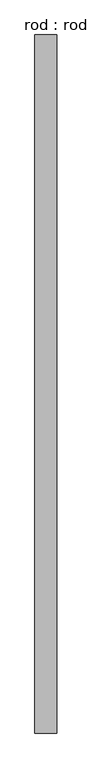
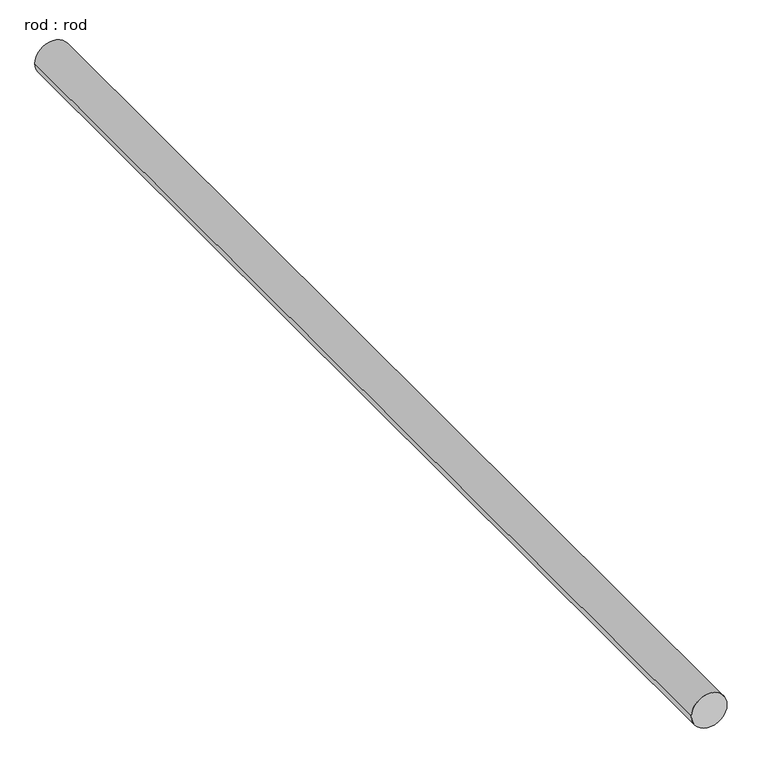
"""IFC4 building model written with IfcOpenShell, lengths in millimetres: proxy geometry, rod : rod."""

from ifc_helpers import new_model, si_unit, point, frame, frame_2d, origin, place, context, project, spatial, circle_curve, trimmed, segment, composite_curve, outline, extrude, source, transform, mapped, element, save


def rod_rod_3cf5adf7(model_context):
    return source(origin(), model_context, "Body", "SweptSolid", [
        extrude(outline(composite_curve([segment(trimmed(circle_curve(frame_2d((0.0108462, 0.0)), 200.0), [point((0.0108462, 200.0))], [point((0.0108462, -200.0))], False, "CARTESIAN"), True, "CONTINUOUS"), segment(trimmed(circle_curve(frame_2d((0.0108462, 0.0)), 200.0), [point((0.0108462, -200.0))], [point((0.0108462, 200.0))], False, "CARTESIAN"), True, "CONTINUOUS")], self_intersect=False)), frame((0.0, -2282.2713847, 0.0), z_axis=(0.0, 1.0, 0.0), x_axis=(0.0, 0.0, 1.0)), (0.0, 0.0, 1.0), 12750.0),
    ])


if __name__ == "__main__":
    model = new_model("IFC4")
    model_context = context("Model", 3, world=origin())
    ifc_project = project(units=[si_unit("LENGTHUNIT", "METRE", prefix="MILLI")], contexts=[model_context])
    site = spatial("IfcSite", under=ifc_project)
    building = spatial("IfcBuilding", under=site)
    placement = place(None, origin())
    rod_rod_shape = rod_rod_3cf5adf7(model_context)
    element("IfcBuildingElementProxy", 1, Name="rod : rod", ObjectType="rod : rod", at=placement, inside=building, context=model_context, shape_type="MappedRepresentation", body=[
        mapped(rod_rod_shape, transform((0.0, 0.0, 0.0), x_axis=(1.0, 0.0, 0.0), y_axis=(0.0, 1.0, 0.0), z_axis=(0.0, 0.0, 1.0))),
    ])
    save(model, "model.ifc")

# Revit data of these elements
# Type "rod : rod"
#   Default Elevation = 0
